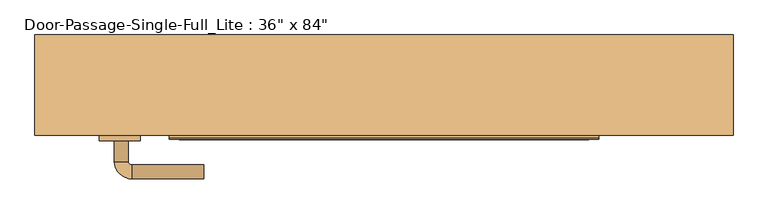
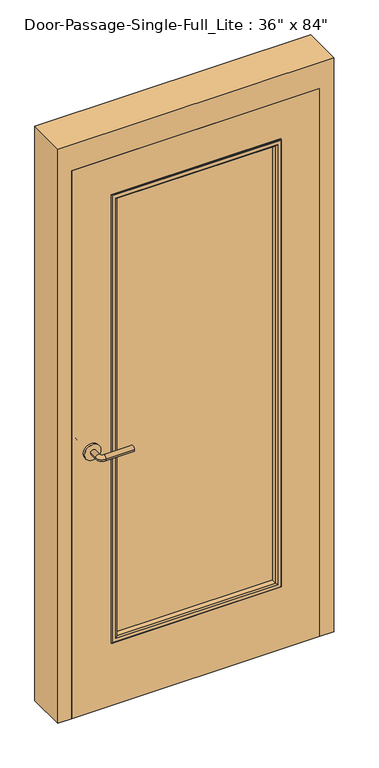
"""IFC4 building model written with IfcOpenShell, lengths in millimetres: door geometry."""

import ifcopenshell
import ifcopenshell.guid

model = None  # the IFC model being written
_history = None  # IfcOwnerHistory: only IFC2X3 demands one
_inside = {}  # id of a spatial element -> (the spatial element, [elements in it])
_under = {}  # id of a project, library or spatial element -> (it, [spatial elements below it])
_declared = {}  # id of a project -> (the project, [libraries it declares])
_typed = {}  # id of a type object -> (the type object, [elements of that type])
_made_of = {}  # id of a material, layer set ... -> (it, [elements and type objects made of it])


def new_model(schema):
    """Start an empty IFC model of exactly this schema.

    Asked for "IFC4X3", IfcOpenShell would pick the latest addendum, in which some entities
    have other attributes; the version numbers below select the first issue.
    IFC2X3 requires an IfcOwnerHistory on every rooted entity: one is made here for all.
    """
    global model, _history
    if schema == "IFC4X3":
        model = ifcopenshell.file(schema_version=(4, 3, 0, 0))
    else:
        model = ifcopenshell.file(schema=schema)
    _inside.clear()
    _under.clear()
    _declared.clear()
    _typed.clear()
    _made_of.clear()
    _history = None
    if model.schema == "IFC2X3":
        org = make("IfcOrganization", Name="unknown")
        user = make(
            "IfcPersonAndOrganization",
            ThePerson=make("IfcPerson", FamilyName="unknown"),
            TheOrganization=org,
        )
        app = make(
            "IfcApplication",
            ApplicationDeveloper=org,
            Version="unknown",
            ApplicationFullName="unknown",
            ApplicationIdentifier="unknown",
        )
        _history = make(
            "IfcOwnerHistory",
            OwningUser=user,
            OwningApplication=app,
            ChangeAction="ADDED",
            CreationDate=0,
        )
    return model


def make(cls, **values):
    """One entity of the class cls with the attributes given. An attribute that is None is left unset."""
    return model.create_entity(
        cls, **{name: value for name, value in values.items() if value is not None}
    )


def rooted(cls, **values):
    """An entity with a GlobalId (a new one), such as an element, a storey or a relation."""
    return make(cls, GlobalId=ifcopenshell.guid.new(), OwnerHistory=_history, **values)


def si_unit(unit_type, name, prefix=None):
    """IfcSIUnit, for example si_unit("LENGTHUNIT", "METRE", prefix="MILLI")."""
    return make("IfcSIUnit", UnitType=unit_type, Prefix=prefix, Name=name)


def assignment(units):
    """IfcUnitAssignment: the units of a project."""
    return None if units is None else make("IfcUnitAssignment", Units=units)


def point(xyz):
    """IfcCartesianPoint."""
    return None if xyz is None else make("IfcCartesianPoint", Coordinates=xyz)


def direction(xyz):
    """IfcDirection."""
    return None if xyz is None else make("IfcDirection", DirectionRatios=xyz)


def frame(location, z_axis=None, x_axis=None):
    """IfcAxis2Placement3D, a coordinate frame: its origin and axes. An axis left out is left unset."""
    return make(
        "IfcAxis2Placement3D",
        Location=point(location),
        Axis=direction(z_axis),
        RefDirection=direction(x_axis),
    )


def frame_2d(location, x_axis=None):
    """IfcAxis2Placement2D, a coordinate frame in the plane: its origin and x axis."""
    return make(
        "IfcAxis2Placement2D", Location=point(location), RefDirection=direction(x_axis)
    )


def origin():
    """The frame at (0, 0, 0) with its axes left unset."""
    return frame((0.0, 0.0, 0.0))


def place(relative_to, where):
    """IfcLocalPlacement: puts the frame where relative to a parent placement (None: the world)."""
    return make(
        "IfcLocalPlacement", PlacementRelTo=relative_to, RelativePlacement=where
    )


def context(
    kind, dimensions, precision=None, world=None, true_north=None, identifier=None
):
    """IfcGeometricRepresentationContext, for example the 3D "Model" context."""
    return make(
        "IfcGeometricRepresentationContext",
        ContextIdentifier=identifier,
        ContextType=kind,
        CoordinateSpaceDimension=dimensions,
        Precision=precision,
        WorldCoordinateSystem=world,
        TrueNorth=true_north,
    )


def project(units=None, contexts=None):
    """IfcProject with its units and contexts."""
    return rooted(
        "IfcProject",
        Name="project",
        RepresentationContexts=contexts,
        UnitsInContext=assignment(units),
    )


def spatial(cls, under=None, at=None, **own):
    """A site, building, storey or space (cls), placed at a placement, below another one or the project."""
    s = rooted(cls, ObjectPlacement=at, **own)
    if under is not None:
        _under.setdefault(under.id(), (under, []))[1].append(s)
    return s


def polyline(points):
    """IfcPolyline through the points."""
    return make("IfcPolyline", Points=[point(p) for p in points])


def circle_curve(where, radius):
    """IfcCircle in the frame where."""
    return make("IfcCircle", Position=where, Radius=radius)


def ellipse_curve(where, semi_axis1, semi_axis2):
    """IfcEllipse in the frame where."""
    return make(
        "IfcEllipse", Position=where, SemiAxis1=semi_axis1, SemiAxis2=semi_axis2
    )


def trimmed(basis, trim1, trim2, sense, master):
    """IfcTrimmedCurve: the piece of a basis curve between two trims."""
    return make(
        "IfcTrimmedCurve",
        BasisCurve=basis,
        Trim1=trim1,
        Trim2=trim2,
        SenseAgreement=sense,
        MasterRepresentation=master,
    )


def segment(curve, same_sense, transition):
    """IfcCompositeCurveSegment."""
    return make(
        "IfcCompositeCurveSegment",
        Transition=transition,
        SameSense=same_sense,
        ParentCurve=curve,
    )


def composite_curve(segments, self_intersect=None):
    """IfcCompositeCurve: segments joined end to end."""
    return make("IfcCompositeCurve", Segments=segments, SelfIntersect=self_intersect)


def outline(outer, holes=None, kind="AREA"):
    """IfcArbitraryClosedProfileDef: a profile drawn as a closed curve; with holes, ...WithVoids."""
    if holes is None:
        return make("IfcArbitraryClosedProfileDef", ProfileType=kind, OuterCurve=outer)
    return make(
        "IfcArbitraryProfileDefWithVoids",
        ProfileType=kind,
        OuterCurve=outer,
        InnerCurves=holes,
    )


def extrude(swept, where, along, depth):
    """IfcExtrudedAreaSolid: the profile swept, set in the frame where, extruded along a direction by depth."""
    return make(
        "IfcExtrudedAreaSolid",
        SweptArea=swept,
        Position=where,
        ExtrudedDirection=direction(along),
        Depth=depth,
    )


def faces_of(points, faces, orient=None, outer=None):
    """IfcFace entities. A face is a list of loops; a loop is a list of indices into points, from 0.

    orient and outer hold one flag for each loop. By default every Orientation is true, the
    first loop of a face is its IfcFaceOuterBound and the others are IfcFaceBound.
    """
    made = []
    for i, loops in enumerate(faces):
        bounds = []
        for j, loop in enumerate(loops):
            is_outer = j == 0 if outer is None else outer[i][j]
            bounds.append(
                make(
                    "IfcFaceOuterBound" if is_outer else "IfcFaceBound",
                    Bound=make("IfcPolyLoop", Polygon=[points[k] for k in loop]),
                    Orientation=True if orient is None else orient[i][j],
                )
            )
        made.append(make("IfcFace", Bounds=bounds))
    return made


def faceted_brep(points, faces, orient=None, outer=None, voids=None):
    """IfcFacetedBrep: a solid bounded by flat faces; with voids (closed shells), ...WithVoids."""
    shared = [point(p) for p in points]
    hull = make("IfcClosedShell", CfsFaces=faces_of(shared, faces, orient, outer))
    if voids is None:
        return make("IfcFacetedBrep", Outer=hull)
    return make(
        "IfcFacetedBrepWithVoids",
        Outer=hull,
        Voids=[
            make(cls, CfsFaces=faces_of(shared, fs, o, b)) for cls, fs, o, b in voids
        ],
    )


def shape(context_of_items, identifier, shape_type, items):
    """IfcShapeRepresentation: the items that make up one representation, for example the "Body"."""
    return make(
        "IfcShapeRepresentation",
        ContextOfItems=context_of_items,
        RepresentationIdentifier=identifier,
        RepresentationType=shape_type,
        Items=items,
    )


def source(mapping_origin, context_of_items, identifier, shape_type, items):
    """IfcRepresentationMap: a shape defined once, which mapped items show again and again."""
    return make(
        "IfcRepresentationMap",
        MappingOrigin=mapping_origin,
        MappedRepresentation=shape(context_of_items, identifier, shape_type, items),
    )


def transform(
    local_origin,
    x_axis=None,
    y_axis=None,
    z_axis=None,
    scale=None,
    scale2=None,
    scale3=None,
    uniform=True,
):
    """IfcCartesianTransformationOperator3D, or its non-uniform kind. x_axis, y_axis, z_axis: its Axis1, 2, 3."""
    if uniform:
        return make(
            "IfcCartesianTransformationOperator3D",
            Axis1=direction(x_axis),
            Axis2=direction(y_axis),
            LocalOrigin=point(local_origin),
            Scale=scale,
            Axis3=direction(z_axis),
        )
    return make(
        "IfcCartesianTransformationOperator3DnonUniform",
        Axis1=direction(x_axis),
        Axis2=direction(y_axis),
        LocalOrigin=point(local_origin),
        Scale=scale,
        Axis3=direction(z_axis),
        Scale2=scale2,
        Scale3=scale3,
    )


def mapped(mapping_source, mapping_target):
    """IfcMappedItem: shows the shape of a source again, moved by a transform."""
    return make(
        "IfcMappedItem", MappingSource=mapping_source, MappingTarget=mapping_target
    )


def made_of(thing, what):
    """Note that an element or type object is made of a material, layer set ...; save() writes the relation."""
    if what is not None:
        _made_of.setdefault(what.id(), (what, []))[1].append(thing)
    return thing


def element(
    cls,
    number,
    at=None,
    inside=None,
    cuts=None,
    type_object=None,
    material=None,
    context=None,
    identifier="Body",
    shape_type=None,
    held_by="IfcProductDefinitionShape",
    body=None,
    shapes=None,
    **own,
):
    """One element of the class cls, such as IfcWall. Its Tag is "e" and its number.

    at: its placement. inside: the storey or other place that contains it. cuts: it is an
    opening in that element (IfcRelVoidsElement). A single representation is given by context,
    identifier, shape_type and body (its items); several are given by shapes. held_by: the class
    of the entity that holds the representations. save() writes the other relations.
    """
    e = rooted(cls, Tag="e%d" % number, ObjectPlacement=at, **own)
    if body is not None:
        shapes = [shape(context, identifier, shape_type, body)]
    if shapes is not None:
        e.Representation = make(held_by, Representations=shapes)
    if inside is not None:
        _inside.setdefault(inside.id(), (inside, []))[1].append(e)
    if cuts is not None:
        rooted(
            "IfcRelVoidsElement", RelatingBuildingElement=cuts, RelatedOpeningElement=e
        )
    if type_object is not None:
        _typed.setdefault(type_object.id(), (type_object, []))[1].append(e)
    return made_of(e, material)


def aggregate(whole, parts):
    """IfcRelAggregates: a whole, such as a stair, and the parts it consists of."""
    return rooted("IfcRelAggregates", RelatingObject=whole, RelatedObjects=parts)


def save(model, path):
    """Write the relations noted so far, then the file.

    IfcRelAggregates (storeys below a building ...), IfcRelContainedInSpatialStructure (elements
    in a storey), IfcRelDefinesByType, IfcRelAssociatesMaterial and IfcRelDeclares: one each for
    every whole, place, type object, material and project.
    """
    for whole, parts in _under.values():
        aggregate(whole, parts)
    for where, things in _inside.values():
        rooted(
            "IfcRelContainedInSpatialStructure",
            RelatedElements=things,
            RelatingStructure=where,
        )
    for kind, things in _typed.values():
        rooted("IfcRelDefinesByType", RelatedObjects=things, RelatingType=kind)
    for what, things in _made_of.values():
        rooted("IfcRelAssociatesMaterial", RelatedObjects=things, RelatingMaterial=what)
    for by, libraries in _declared.values():
        rooted("IfcRelDeclares", RelatingContext=by, RelatedDefinitions=libraries)
    model.write(path)


def plane_surface(at):
    """IfcPlane: the flat surface through the origin of the frame at, square to its z axis."""
    return make("IfcPlane", Position=at)


def cylinder_surface(at, radius):
    """IfcCylindricalSurface: all points at the distance radius from the z axis of the frame at."""
    return make("IfcCylindricalSurface", Position=at, Radius=radius)


def revolved_surface(curve, axis_point, axis_direction):
    """IfcSurfaceOfRevolution: the curve turned about the line through axis_point along axis_direction."""
    return make(
        "IfcSurfaceOfRevolution",
        SweptCurve=make("IfcArbitraryOpenProfileDef", ProfileType="CURVE", Curve=curve),
        AxisPosition=make("IfcAxis1Placement", Location=point(axis_point), Axis=direction(axis_direction)),
    )


def advanced_brep(points, edges, surfaces, faces):
    """IfcAdvancedBrep: a solid bounded by faces that lie on surfaces and meet in shared edges.

    An edge is (start, end): straight between two places in points (the first is 0);
    or (start, end, curve); or (start, end, curve, False) where it runs against its curve.
    A face is (place in surfaces, loops), or (place, loops, False) where it looks against
    its surface's normal. A loop lists edges by number (the first is 1), with a minus sign
    where the edge is run from its end to its start. The first loop is the outer one.
    """
    corners = [point(p) for p in points]
    vertices = [make("IfcVertexPoint", VertexGeometry=c) for c in corners]
    made = []
    for start, end, *more in edges:
        made.append(
            make(
                "IfcEdgeCurve",
                EdgeStart=vertices[start],
                EdgeEnd=vertices[end],
                EdgeGeometry=more[0] if more else make("IfcPolyline", Points=[corners[start], corners[end]]),
                SameSense=more[1] if len(more) > 1 else True,
            )
        )
    hull = []
    for where, loops, *sense in faces:
        bounds = []
        for j, loop in enumerate(loops):
            ring = [make("IfcOrientedEdge", EdgeElement=made[abs(k) - 1], Orientation=k > 0) for k in loop]
            bounds.append(
                make(
                    "IfcFaceOuterBound" if j == 0 else "IfcFaceBound",
                    Bound=make("IfcEdgeLoop", EdgeList=ring),
                    Orientation=True,
                )
            )
        hull.append(make("IfcAdvancedFace", Bounds=bounds, FaceSurface=surfaces[where], SameSense=sense[0] if sense else True))
    return make("IfcAdvancedBrep", Outer=make("IfcClosedShell", CfsFaces=hull))


def door_5fc50167(model_context):
    return source(origin(), model_context, "Body", "SolidModel", [
        advanced_brep(
        [(-392.190625, 9.5875, 1016.0), (-372.190625, 9.5875, 1016.0), (-392.190625, 39.5875, 1016.0), (-372.190625, 39.5875, 1016.0), (-367.190625, 44.5875, 1016.0), (-367.190625, 64.5875, 1016.0), (-262.190625, 64.5875, 1016.0), (-262.190625, 44.5875, 1016.0)],
        [
            (0, 1, circle_curve(frame((-382.190625, 9.5875, 1016.0), z_axis=(0.0, -1.0, 0.0), x_axis=(1.0, 0.0, 0.0)), 10.0)),
            (1, 0, circle_curve(frame((-382.190625, 9.5875, 1016.0), z_axis=(0.0, -1.0, 0.0), x_axis=(1.0, 0.0, 0.0)), 10.0)),
            (0, 2),
            (2, 3, circle_curve(frame((-382.190625, 39.5875, 1016.0), z_axis=(0.0, -1.0, 0.0), x_axis=(1.0, 0.0, 0.0)), 10.0)),
            (3, 1),
            (3, 2, circle_curve(frame((-382.190625, 39.5875, 1016.0), z_axis=(0.0, -1.0, 0.0), x_axis=(1.0, 0.0, 0.0)), 10.0)),
            (4, 3, circle_curve(frame((-367.190625, 39.5875, 1016.0), z_axis=(0.0, 0.0, 1.0), x_axis=(-1.0, 0.0, 0.0)), 5.0)),
            (2, 5, circle_curve(frame((-367.190625, 39.5875, 1016.0), z_axis=(0.0, 0.0, -1.0), x_axis=(-1.0, 0.0, 0.0)), 25.0)),
            (5, 4, circle_curve(frame((-367.190625, 54.5875, 1016.0), z_axis=(-1.0, 0.0, 0.0), x_axis=(0.0, -1.0, 0.0)), 10.0)),
            (4, 5, circle_curve(frame((-367.190625, 54.5875, 1016.0), z_axis=(-1.0, 0.0, 0.0), x_axis=(0.0, -1.0, 0.0)), 10.0)),
            (6, 7, circle_curve(frame((-262.190625, 54.5875, 1016.0), z_axis=(1.0, 0.0, 0.0), x_axis=(0.0, -1.0, 0.0)), 10.0)),
            (7, 6, circle_curve(frame((-262.190625, 54.5875, 1016.0), z_axis=(1.0, 0.0, 0.0), x_axis=(0.0, -1.0, 0.0)), 10.0)),
            (5, 6),
            (7, 4),
        ],
        [
            plane_surface(frame((-382.190625, 9.5875, 1016.0), z_axis=(0.0, -1.0, 0.0), x_axis=(0.0, 0.0, 1.0))),
            cylinder_surface(frame((-382.190625, 9.5875, 1016.0), z_axis=(0.0, -1.0, 0.0), x_axis=(1.0, 0.0, 0.0)), 10.0),
            revolved_surface(trimmed(ellipse_curve(frame((-382.190625, 39.5875, 1016.0), z_axis=(0.0, -1.0, 0.0), x_axis=(1.0, 0.0, 0.0)), 10.0, 10.0), [point((-392.190625, 39.5875, 1016.0))], [point((-372.190625, 39.5875, 1016.0))], True, "CARTESIAN"), (-367.190625, 39.5875, 1016.0), (0.0, 0.0, -1.0)),
            revolved_surface(trimmed(ellipse_curve(frame((-382.190625, 39.5875, 1016.0), z_axis=(0.0, -1.0, 0.0), x_axis=(1.0, 0.0, 0.0)), 10.0, 10.0), [point((-372.190625, 39.5875, 1016.0))], [point((-392.190625, 39.5875, 1016.0))], True, "CARTESIAN"), (-367.190625, 39.5875, 1016.0), (0.0, 0.0, -1.0)),
            plane_surface(frame((-262.190625, 54.5875, 1016.0), z_axis=(1.0, 0.0, 0.0), x_axis=(0.0, 0.0, 1.0))),
            cylinder_surface(frame((-367.190625, 54.5875, 1016.0), z_axis=(-1.0, 0.0, 0.0), x_axis=(0.0, -1.0, 0.0)), 10.0),
        ],
        [
            (0, [[1, 2]]),
            (1, [[-1, 3, 4, 5]]),
            (1, [[-2, -5, 6, -3]]),
            (2, [[7, -4, 8, 9]]),
            (3, [[-8, -6, -7, 10]]),
            (4, [[11, 12]]),
            (5, [[-9, 13, -12, 14]]),
            (5, [[-10, -14, -11, -13]]),
        ],
    ),
        extrude(outline(composite_curve([segment(trimmed(circle_curve(frame_2d((1016.0, -384.690625)), 30.0), [point((1016.0, -414.690625))], [point((1016.0, -354.690625))], False, "CARTESIAN"), True, "CONTINUOUS"), segment(trimmed(circle_curve(frame_2d((1016.0, -384.690625)), 30.0), [point((1016.0, -354.690625))], [point((1016.0, -414.690625))], False, "CARTESIAN"), True, "CONTINUOUS")], self_intersect=False)), frame((0.0, 1.5875, 0.0), z_axis=(0.0, 1.0, 0.0), x_axis=(0.0, 0.0, 1.0)), (0.0, 0.0, 1.0), 8.0),
        advanced_brep(
        [(-392.190625, -50.8625, 1016.0), (-372.190625, -50.8625, 1016.0), (-372.190625, -80.8625, 1016.0), (-392.190625, -80.8625, 1016.0), (-367.190625, -85.8625, 1016.0), (-367.190625, -105.8625, 1016.0), (-262.190625, -105.8625, 1016.0), (-262.190625, -85.8625, 1016.0)],
        [
            (0, 1, circle_curve(frame((-382.190625, -50.8625, 1016.0), z_axis=(0.0, 1.0, 0.0), x_axis=(1.0, 0.0, 0.0)), 10.0)),
            (1, 0, circle_curve(frame((-382.190625, -50.8625, 1016.0), z_axis=(0.0, 1.0, 0.0), x_axis=(1.0, 0.0, 0.0)), 10.0)),
            (1, 2),
            (2, 3, circle_curve(frame((-382.190625, -80.8625, 1016.0), z_axis=(0.0, 1.0, 0.0), x_axis=(1.0, 0.0, 0.0)), 10.0)),
            (3, 0),
            (3, 2, circle_curve(frame((-382.190625, -80.8625, 1016.0), z_axis=(0.0, 1.0, 0.0), x_axis=(1.0, 0.0, 0.0)), 10.0)),
            (4, 5, circle_curve(frame((-367.190625, -95.8625, 1016.0), z_axis=(-1.0, 0.0, 0.0), x_axis=(0.0, 1.0, 0.0)), 10.0)),
            (5, 3, circle_curve(frame((-367.190625, -80.8625, 1016.0), z_axis=(0.0, 0.0, -1.0), x_axis=(-1.0, 0.0, 0.0)), 25.0)),
            (2, 4, circle_curve(frame((-367.190625, -80.8625, 1016.0), z_axis=(0.0, 0.0, 1.0), x_axis=(-1.0, 0.0, 0.0)), 5.0)),
            (5, 4, circle_curve(frame((-367.190625, -95.8625, 1016.0), z_axis=(-1.0, 0.0, 0.0), x_axis=(0.0, 1.0, 0.0)), 10.0)),
            (6, 7, circle_curve(frame((-262.190625, -95.8625, 1016.0), z_axis=(1.0, 0.0, 0.0), x_axis=(0.0, 1.0, 0.0)), 10.0)),
            (7, 6, circle_curve(frame((-262.190625, -95.8625, 1016.0), z_axis=(1.0, 0.0, 0.0), x_axis=(0.0, 1.0, 0.0)), 10.0)),
            (4, 7),
            (6, 5),
        ],
        [
            plane_surface(frame((-382.190625, -50.8625, 1016.0), z_axis=(0.0, 1.0, 0.0), x_axis=(0.0, 0.0, 1.0))),
            cylinder_surface(frame((-382.190625, -50.8625, 1016.0), z_axis=(0.0, 1.0, 0.0), x_axis=(1.0, 0.0, 0.0)), 10.0),
            revolved_surface(trimmed(ellipse_curve(frame((-382.190625, -80.8625, 1016.0), z_axis=(0.0, -1.0, 0.0), x_axis=(1.0, 0.0, 0.0)), 10.0, 10.0), [point((-392.190625, -80.8625, 1016.0))], [point((-372.190625, -80.8625, 1016.0))], True, "CARTESIAN"), (-367.190625, -80.8625, 1016.0), (0.0, 0.0, -1.0)),
            revolved_surface(trimmed(ellipse_curve(frame((-382.190625, -80.8625, 1016.0), z_axis=(0.0, -1.0, 0.0), x_axis=(1.0, 0.0, 0.0)), 10.0, 10.0), [point((-372.190625, -80.8625, 1016.0))], [point((-392.190625, -80.8625, 1016.0))], True, "CARTESIAN"), (-367.190625, -80.8625, 1016.0), (0.0, 0.0, -1.0)),
            plane_surface(frame((-262.190625, -95.8625, 1016.0), z_axis=(1.0, 0.0, 0.0), x_axis=(0.0, 0.0, 1.0))),
            cylinder_surface(frame((-367.190625, -95.8625, 1016.0), z_axis=(-1.0, 0.0, 0.0), x_axis=(0.0, 1.0, 0.0)), 10.0),
        ],
        [
            (0, [[1, 2]]),
            (1, [[3, 4, 5, -2]]),
            (1, [[-5, 6, -3, -1]]),
            (2, [[7, 8, -4, 9]]),
            (3, [[10, -9, -6, -8]]),
            (4, [[11, 12]]),
            (5, [[13, -11, 14, -7]]),
            (5, [[-14, -12, -13, -10]]),
        ],
    ),
        extrude(outline(composite_curve([segment(trimmed(circle_curve(frame_2d((1016.0, -384.690625)), 30.0), [point((1016.0, -414.690625))], [point((1016.0, -354.690625))], False, "CARTESIAN"), True, "CONTINUOUS"), segment(trimmed(circle_curve(frame_2d((1016.0, -384.690625)), 30.0), [point((1016.0, -354.690625))], [point((1016.0, -414.690625))], False, "CARTESIAN"), True, "CONTINUOUS")], self_intersect=False)), frame((0.0, -50.8625, 0.0), z_axis=(0.0, 1.0, 0.0), x_axis=(0.0, 0.0, 1.0)), (0.0, 0.0, 1.0), 8.0),
        extrude(outline(polyline([(304.8, -17.4625), (304.8, -23.8125), (-304.8, -23.8125), (-304.8, -17.4625), (304.8, -17.4625)])), frame((0.0, 0.0, 254.0), z_axis=(0.0, 0.0, 1.0), x_axis=(1.0, 0.0, 0.0)), (0.0, 0.0, 1.0), 1727.2),
        faceted_brep([(457.2, 6.35, 0.0), (441.325, 6.35, 0.0), (441.325, 53.975, 0.0), (457.2, 53.975, 0.0), (457.2, 103.1875, 0.0), (508.0, 103.1875, 0.0), (508.0, -42.8625, 0.0), (457.2, -42.8625, 0.0), (457.2, -42.8625, 2133.6), (457.2, 6.35, 2133.6), (508.0, -42.8625, 2235.2), (-508.0, -42.8625, 2235.2), (-508.0, -42.8625, 0.0), (-457.2, -42.8625, 0.0), (-457.2, -42.8625, 2133.6), (508.0, 103.1875, 2235.2), (457.2, 103.1875, 2133.6), (-457.2, 103.1875, 2133.6), (-457.2, 103.1875, 0.0), (-508.0, 103.1875, 0.0), (-508.0, 103.1875, 2235.2), (457.2, 53.975, 2133.6), (441.325, 53.975, 2117.725), (-441.325, 53.975, 2117.725), (-441.325, 53.975, 0.0), (-457.2, 53.975, 0.0), (-457.2, 53.975, 2133.6), (441.325, 6.35, 2117.725), (-457.2, 6.35, 2133.6), (-457.2, 6.35, 0.0), (-441.325, 6.35, 0.0), (-441.325, 6.35, 2117.725)], [[[0, 1, 2, 3, 4, 5, 6, 7]], [[7, 8, 9, 0]], [[6, 10, 11, 12, 13, 14, 8, 7]], [[5, 15, 10, 6]], [[4, 16, 17, 18, 19, 20, 15, 5]], [[3, 21, 16, 4]], [[2, 22, 23, 24, 25, 26, 21, 3]], [[1, 27, 22, 2]], [[0, 9, 28, 29, 30, 31, 27, 1]], [[8, 14, 28, 9]], [[16, 21, 26, 17]], [[22, 27, 31, 23]], [[12, 19, 18, 25, 24, 30, 29, 13]], [[13, 29, 28, 14]], [[11, 20, 19, 12]], [[17, 26, 25, 18]], [[23, 31, 30, 24]], [[15, 20, 11, 10]]]),
        extrude(outline(polyline([(2133.6, -457.2), (0.0, -457.2), (0.0, 457.2), (2133.6, 457.2), (2133.6, -457.2)]), holes=[polyline([(1981.2, -304.8), (1981.2, 304.8), (254.0, 304.8), (254.0, -304.8), (1981.2, -304.8)])]), frame((0.0, -42.8625, 0.0), z_axis=(0.0, 1.0, 0.0), x_axis=(0.0, 0.0, 1.0)), (0.0, 0.0, 1.0), 44.45),
        advanced_brep(
        [(-304.8, -23.8125, 1981.2), (-304.8, -23.8125, 254.0), (-304.8, -42.8625, 254.0), (-304.8, -42.8625, 1981.2), (-292.8, -43.8625, 1969.2), (-292.8, -43.8625, 266.0), (-292.8, -23.8125, 266.0), (-292.8, -23.8125, 1969.2), (-297.8, -48.8625, 1974.2), (-297.8, -48.8625, 261.0), (-312.8, -46.8625, 1989.2), (-312.8, -46.8625, 246.0), (-310.8, -48.8625, 248.0), (-310.8, -48.8625, 1987.2), (-312.8, -42.8625, 1989.2), (-312.8, -42.8625, 246.0), (304.8, -23.8125, 254.0), (304.8, -42.8625, 254.0), (292.8, -43.8625, 266.0), (292.8, -23.8125, 266.0), (297.8, -48.8625, 261.0), (312.8, -46.8625, 246.0), (310.8, -48.8625, 248.0), (312.8, -42.8625, 246.0), (304.8, -23.8125, 1981.2), (304.8, -42.8625, 1981.2), (292.8, -43.8625, 1969.2), (292.8, -23.8125, 1969.2), (297.8, -48.8625, 1974.2), (312.8, -46.8625, 1989.2), (310.8, -48.8625, 1987.2), (312.8, -42.8625, 1989.2)],
        [
            (0, 1),
            (1, 2),
            (2, 3),
            (3, 0),
            (4, 5),
            (5, 6),
            (6, 7),
            (7, 4),
            (8, 9),
            (9, 5, ellipse_curve(frame((-297.8, -43.8625, 261.0), z_axis=(-0.7071067811865475, 0.0, 0.7071067811865475), x_axis=(0.7071067811865474, 0.0, 0.7071067811865476)), 7.0710678, 5.0)),
            (4, 8, ellipse_curve(frame((-297.8, -43.8625, 1974.2), z_axis=(-0.7071067811865475, 0.0, -0.7071067811865475), x_axis=(-0.7071067811865474, 0.0, 0.7071067811865476)), 7.0710678, 5.0)),
            (10, 11),
            (11, 12, ellipse_curve(frame((-310.8, -46.8625, 248.0), z_axis=(-0.7071067811865475, 0.0, 0.7071067811865475), x_axis=(0.7071067811865474, 0.0, 0.7071067811865476)), 2.8284271, 2.0)),
            (12, 13),
            (13, 10, ellipse_curve(frame((-310.8, -46.8625, 1987.2), z_axis=(-0.7071067811865475, 0.0, -0.7071067811865475), x_axis=(-0.7071067811865474, 0.0, 0.7071067811865476)), 2.8284271, 2.0)),
            (14, 15),
            (15, 11),
            (10, 14),
            (1, 16),
            (16, 17),
            (17, 2),
            (5, 18),
            (18, 19),
            (19, 6),
            (9, 20),
            (20, 18, ellipse_curve(frame((297.8, -43.8625, 261.0), z_axis=(-0.7071067811865475, 0.0, -0.7071067811865475), x_axis=(-0.7071067811865476, 0.0, 0.7071067811865474)), 7.0710678, 5.0)),
            (11, 21),
            (21, 22, ellipse_curve(frame((310.8, -46.8625, 248.0), z_axis=(-0.7071067811865475, 0.0, -0.7071067811865475), x_axis=(-0.7071067811865476, 0.0, 0.7071067811865474)), 2.8284271, 2.0)),
            (22, 12),
            (15, 23),
            (23, 21),
            (16, 24),
            (24, 25),
            (25, 17),
            (18, 26),
            (26, 27),
            (27, 19),
            (20, 28),
            (28, 26, ellipse_curve(frame((297.8, -43.8625, 1974.2), z_axis=(0.7071067811865475, 0.0, -0.7071067811865475), x_axis=(-0.7071067811865474, 0.0, -0.7071067811865476)), 7.0710678, 5.0)),
            (21, 29),
            (29, 30, ellipse_curve(frame((310.8, -46.8625, 1987.2), z_axis=(0.7071067811865475, 0.0, -0.7071067811865475), x_axis=(-0.7071067811865474, 0.0, -0.7071067811865476)), 2.8284271, 2.0)),
            (30, 22),
            (23, 31),
            (31, 29),
            (14, 31),
            (25, 3),
            (24, 0),
            (27, 7),
            (26, 4),
            (28, 8),
            (30, 13),
            (29, 10),
        ],
        [
            plane_surface(frame((-304.8, -42.8625, 1981.2), z_axis=(-1.0, 0.0, 0.0), x_axis=(0.0, 0.0, -1.0))),
            plane_surface(frame((-292.8, -23.8125, 1969.2), z_axis=(1.0, 0.0, 0.0), x_axis=(0.0, 0.0, -1.0))),
            cylinder_surface(frame((-297.8, -43.8625, 1981.2), z_axis=(0.0, 0.0, 1.0), x_axis=(-1.0, 0.0, 0.0)), 5.0),
            cylinder_surface(frame((-310.8, -46.8625, 1981.2), z_axis=(0.0, 0.0, 1.0), x_axis=(-1.0, 0.0, 0.0)), 2.0),
            plane_surface(frame((-312.8, -46.8625, 1989.2), z_axis=(-1.0, 0.0, 0.0), x_axis=(0.0, 0.0, -1.0))),
            plane_surface(frame((-304.8, -42.8625, 254.0), z_axis=(0.0, 0.0, -1.0), x_axis=(1.0, 0.0, 0.0))),
            plane_surface(frame((-292.8, -23.8125, 266.0), z_axis=(0.0, 0.0, 1.0), x_axis=(1.0, 0.0, 0.0))),
            cylinder_surface(frame((-304.8, -43.8625, 261.0), z_axis=(-1.0, 0.0, 0.0), x_axis=(0.0, 0.0, -1.0)), 5.0),
            cylinder_surface(frame((-304.8, -46.8625, 248.0), z_axis=(-1.0, 0.0, 0.0), x_axis=(0.0, 0.0, -1.0)), 2.0),
            plane_surface(frame((-312.8, -46.8625, 246.0), z_axis=(0.0, 0.0, -1.0), x_axis=(1.0, 0.0, 0.0))),
            plane_surface(frame((304.8, -42.8625, 254.0), z_axis=(1.0, 0.0, 0.0), x_axis=(0.0, 0.0, 1.0))),
            plane_surface(frame((292.8, -23.8125, 266.0), z_axis=(-1.0, 0.0, 0.0), x_axis=(0.0, 0.0, 1.0))),
            cylinder_surface(frame((297.8, -43.8625, 254.0), z_axis=(0.0, 0.0, -1.0), x_axis=(1.0, 0.0, 0.0)), 5.0),
            cylinder_surface(frame((310.8, -46.8625, 254.0), z_axis=(0.0, 0.0, -1.0), x_axis=(1.0, 0.0, 0.0)), 2.0),
            plane_surface(frame((312.8, -46.8625, 246.0), z_axis=(1.0, 0.0, 0.0), x_axis=(0.0, 0.0, 1.0))),
            plane_surface(frame((312.8, -42.8625, 1989.2), z_axis=(0.0, 1.0, 0.0), x_axis=(-1.0, 0.0, 0.0))),
            plane_surface(frame((304.8, -42.8625, 1981.2), z_axis=(0.0, 0.0, 1.0), x_axis=(-1.0, 0.0, 0.0))),
            plane_surface(frame((304.8, -23.8125, 1981.2), z_axis=(0.0, 1.0, 0.0), x_axis=(-1.0, 0.0, 0.0))),
            plane_surface(frame((292.8, -23.8125, 1969.2), z_axis=(0.0, 0.0, -1.0), x_axis=(-1.0, 0.0, 0.0))),
            cylinder_surface(frame((304.8, -43.8625, 1974.2), z_axis=(1.0, 0.0, 0.0), x_axis=(0.0, 0.0, 1.0)), 5.0),
            plane_surface(frame((297.8, -48.8625, 1974.2), z_axis=(0.0, -1.0, 0.0), x_axis=(-1.0, 0.0, 0.0))),
            cylinder_surface(frame((304.8, -46.8625, 1987.2), z_axis=(1.0, 0.0, 0.0), x_axis=(0.0, 0.0, 1.0)), 2.0),
            plane_surface(frame((312.8, -46.8625, 1989.2), z_axis=(0.0, 0.0, 1.0), x_axis=(-1.0, 0.0, 0.0))),
        ],
        [
            (0, [[1, 2, 3, 4]]),
            (1, [[5, 6, 7, 8]]),
            (2, [[9, 10, -5, 11]]),
            (3, [[12, 13, 14, 15]]),
            (4, [[16, 17, -12, 18]]),
            (5, [[19, 20, 21, -2]]),
            (6, [[22, 23, 24, -6]]),
            (7, [[25, 26, -22, -10]]),
            (8, [[27, 28, 29, -13]]),
            (9, [[30, 31, -27, -17]]),
            (10, [[32, 33, 34, -20]]),
            (11, [[35, 36, 37, -23]]),
            (12, [[38, 39, -35, -26]]),
            (13, [[40, 41, 42, -28]]),
            (14, [[43, 44, -40, -31]]),
            (15, [[-16, 45, -43, -30], [-3, -21, -34, 46]]),
            (16, [[47, -4, -46, -33]]),
            (17, [[-1, -47, -32, -19], [-7, -24, -37, 48]]),
            (18, [[49, -8, -48, -36]]),
            (19, [[50, -11, -49, -39]]),
            (20, [[-14, -29, -42, 51], [-9, -50, -38, -25]]),
            (21, [[52, -15, -51, -41]]),
            (22, [[-45, -18, -52, -44]]),
        ],
    ),
        advanced_brep(
        [(-304.8, -17.4625, 254.0), (-304.8, -17.4625, 1981.2), (-304.8, 1.5875, 1981.2), (-304.8, 1.5875, 254.0), (-292.8, 2.5875, 266.0), (-292.8, 2.5875, 1969.2), (-292.8, -17.4625, 1969.2), (-292.8, -17.4625, 266.0), (-297.8, 7.5875, 261.0), (-297.8, 7.5875, 1974.2), (-312.8, 5.5875, 246.0), (-312.8, 5.5875, 1989.2), (-310.8, 7.5875, 1987.2), (-310.8, 7.5875, 248.0), (-312.8, 1.5875, 246.0), (-312.8, 1.5875, 1989.2), (304.8, -17.4625, 1981.2), (304.8, 1.5875, 1981.2), (292.8, 2.5875, 1969.2), (292.8, -17.4625, 1969.2), (297.8, 7.5875, 1974.2), (312.8, 5.5875, 1989.2), (310.8, 7.5875, 1987.2), (312.8, 1.5875, 1989.2), (304.8, -17.4625, 254.0), (304.8, 1.5875, 254.0), (292.8, 2.5875, 266.0), (292.8, -17.4625, 266.0), (297.8, 7.5875, 261.0), (312.8, 5.5875, 246.0), (310.8, 7.5875, 248.0), (312.8, 1.5875, 246.0)],
        [
            (0, 1),
            (1, 2),
            (2, 3),
            (3, 0),
            (4, 5),
            (5, 6),
            (6, 7),
            (7, 4),
            (8, 9),
            (9, 5, ellipse_curve(frame((-297.8, 2.5875, 1974.2), z_axis=(-0.7071067811865475, 0.0, -0.7071067811865475), x_axis=(0.7071067811865474, 0.0, -0.7071067811865476)), 7.0710678, 5.0)),
            (4, 8, ellipse_curve(frame((-297.8, 2.5875, 261.0), z_axis=(-0.7071067811865475, 0.0, 0.7071067811865475), x_axis=(-0.7071067811865474, 0.0, -0.7071067811865476)), 7.0710678, 5.0)),
            (10, 11),
            (11, 12, ellipse_curve(frame((-310.8, 5.5875, 1987.2), z_axis=(-0.7071067811865475, 0.0, -0.7071067811865475), x_axis=(0.7071067811865474, 0.0, -0.7071067811865476)), 2.8284271, 2.0)),
            (12, 13),
            (13, 10, ellipse_curve(frame((-310.8, 5.5875, 248.0), z_axis=(-0.7071067811865475, 0.0, 0.7071067811865475), x_axis=(-0.7071067811865474, 0.0, -0.7071067811865476)), 2.8284271, 2.0)),
            (14, 15),
            (15, 11),
            (10, 14),
            (1, 16),
            (16, 17),
            (17, 2),
            (5, 18),
            (18, 19),
            (19, 6),
            (9, 20),
            (20, 18, ellipse_curve(frame((297.8, 2.5875, 1974.2), z_axis=(-0.7071067811865475, 0.0, 0.7071067811865475), x_axis=(-0.7071067811865476, 0.0, -0.7071067811865474)), 7.0710678, 5.0)),
            (11, 21),
            (21, 22, ellipse_curve(frame((310.8, 5.5875, 1987.2), z_axis=(-0.7071067811865475, 0.0, 0.7071067811865475), x_axis=(-0.7071067811865476, 0.0, -0.7071067811865474)), 2.8284271, 2.0)),
            (22, 12),
            (15, 23),
            (23, 21),
            (16, 24),
            (24, 25),
            (25, 17),
            (18, 26),
            (26, 27),
            (27, 19),
            (20, 28),
            (28, 26, ellipse_curve(frame((297.8, 2.5875, 261.0), z_axis=(0.7071067811865475, 0.0, 0.7071067811865475), x_axis=(-0.7071067811865474, 0.0, 0.7071067811865476)), 7.0710678, 5.0)),
            (21, 29),
            (29, 30, ellipse_curve(frame((310.8, 5.5875, 248.0), z_axis=(0.7071067811865475, 0.0, 0.7071067811865475), x_axis=(-0.7071067811865474, 0.0, 0.7071067811865476)), 2.8284271, 2.0)),
            (30, 22),
            (23, 31),
            (31, 29),
            (14, 31),
            (25, 3),
            (24, 0),
            (27, 7),
            (26, 4),
            (28, 8),
            (30, 13),
            (29, 10),
        ],
        [
            plane_surface(frame((-304.8, 1.5875, 254.0), z_axis=(-1.0, 0.0, 0.0), x_axis=(0.0, 0.0, 1.0))),
            plane_surface(frame((-292.8, -17.4625, 266.0), z_axis=(1.0, 0.0, 0.0), x_axis=(0.0, 0.0, 1.0))),
            cylinder_surface(frame((-297.8, 2.5875, 254.0), z_axis=(0.0, 0.0, -1.0), x_axis=(-1.0, 0.0, 0.0)), 5.0),
            cylinder_surface(frame((-310.8, 5.5875, 254.0), z_axis=(0.0, 0.0, -1.0), x_axis=(-1.0, 0.0, 0.0)), 2.0),
            plane_surface(frame((-312.8, 5.5875, 246.0), z_axis=(-1.0, 0.0, 0.0), x_axis=(0.0, 0.0, 1.0))),
            plane_surface(frame((-304.8, 1.5875, 1981.2), z_axis=(0.0, 0.0, 1.0), x_axis=(1.0, 0.0, 0.0))),
            plane_surface(frame((-292.8, -17.4625, 1969.2), z_axis=(0.0, 0.0, -1.0), x_axis=(1.0, 0.0, 0.0))),
            cylinder_surface(frame((-304.8, 2.5875, 1974.2), z_axis=(-1.0, 0.0, 0.0), x_axis=(0.0, 0.0, 1.0)), 5.0),
            cylinder_surface(frame((-304.8, 5.5875, 1987.2), z_axis=(-1.0, 0.0, 0.0), x_axis=(0.0, 0.0, 1.0)), 2.0),
            plane_surface(frame((-312.8, 5.5875, 1989.2), z_axis=(0.0, 0.0, 1.0), x_axis=(1.0, 0.0, 0.0))),
            plane_surface(frame((304.8, 1.5875, 1981.2), z_axis=(1.0, 0.0, 0.0), x_axis=(0.0, 0.0, -1.0))),
            plane_surface(frame((292.8, -17.4625, 1969.2), z_axis=(-1.0, 0.0, 0.0), x_axis=(0.0, 0.0, -1.0))),
            cylinder_surface(frame((297.8, 2.5875, 1981.2), z_axis=(0.0, 0.0, 1.0), x_axis=(1.0, 0.0, 0.0)), 5.0),
            cylinder_surface(frame((310.8, 5.5875, 1981.2), z_axis=(0.0, 0.0, 1.0), x_axis=(1.0, 0.0, 0.0)), 2.0),
            plane_surface(frame((312.8, 5.5875, 1989.2), z_axis=(1.0, 0.0, 0.0), x_axis=(0.0, 0.0, -1.0))),
            plane_surface(frame((312.8, 1.5875, 246.0), z_axis=(0.0, -1.0, 0.0), x_axis=(-1.0, 0.0, 0.0))),
            plane_surface(frame((304.8, 1.5875, 254.0), z_axis=(0.0, 0.0, -1.0), x_axis=(-1.0, 0.0, 0.0))),
            plane_surface(frame((304.8, -17.4625, 254.0), z_axis=(0.0, -1.0, 0.0), x_axis=(-1.0, 0.0, 0.0))),
            plane_surface(frame((292.8, -17.4625, 266.0), z_axis=(0.0, 0.0, 1.0), x_axis=(-1.0, 0.0, 0.0))),
            cylinder_surface(frame((304.8, 2.5875, 261.0), z_axis=(1.0, 0.0, 0.0), x_axis=(0.0, 0.0, -1.0)), 5.0),
            plane_surface(frame((297.8, 7.5875, 261.0), z_axis=(0.0, 1.0, 0.0), x_axis=(-1.0, 0.0, 0.0))),
            cylinder_surface(frame((304.8, 5.5875, 248.0), z_axis=(1.0, 0.0, 0.0), x_axis=(0.0, 0.0, -1.0)), 2.0),
            plane_surface(frame((312.8, 5.5875, 246.0), z_axis=(0.0, 0.0, -1.0), x_axis=(-1.0, 0.0, 0.0))),
        ],
        [
            (0, [[1, 2, 3, 4]]),
            (1, [[5, 6, 7, 8]]),
            (2, [[9, 10, -5, 11]]),
            (3, [[12, 13, 14, 15]]),
            (4, [[16, 17, -12, 18]]),
            (5, [[19, 20, 21, -2]]),
            (6, [[22, 23, 24, -6]]),
            (7, [[25, 26, -22, -10]]),
            (8, [[27, 28, 29, -13]]),
            (9, [[30, 31, -27, -17]]),
            (10, [[32, 33, 34, -20]]),
            (11, [[35, 36, 37, -23]]),
            (12, [[38, 39, -35, -26]]),
            (13, [[40, 41, 42, -28]]),
            (14, [[43, 44, -40, -31]]),
            (15, [[-16, 45, -43, -30], [-3, -21, -34, 46]]),
            (16, [[47, -4, -46, -33]]),
            (17, [[-1, -47, -32, -19], [-7, -24, -37, 48]]),
            (18, [[49, -8, -48, -36]]),
            (19, [[50, -11, -49, -39]]),
            (20, [[-14, -29, -42, 51], [-9, -50, -38, -25]]),
            (21, [[52, -15, -51, -41]]),
            (22, [[-45, -18, -52, -44]]),
        ],
    ),
    ])


if __name__ == "__main__":
    model = new_model("IFC4")
    model_context = context("Model", 3, world=origin())
    ifc_project = project(units=[si_unit("LENGTHUNIT", "METRE", prefix="MILLI")], contexts=[model_context])
    site = spatial("IfcSite", under=ifc_project)
    building = spatial("IfcBuilding", under=site)
    placement = place(None, origin())
    door_shape = door_5fc50167(model_context)
    element("IfcDoor", 1, ObjectType="Door-Passage-Single-Full_Lite : 36\" x 84\"", at=placement, inside=building, context=model_context, shape_type="MappedRepresentation", body=[
        mapped(door_shape, transform((0.0, 0.0, 0.0), x_axis=(1.0, 0.0, 0.0), y_axis=(0.0, 1.0, 0.0), z_axis=(0.0, 0.0, 1.0))),
    ])
    save(model, "model.ifc")

# Revit data of these elements
# Type "Door-Passage-Single-Full_Lite : 36\" x 84\""
#   Type Mark = "52"
#   Assembly Code = "B2030100"
#   Analytic Construction = "Wooden"
#   Thickness = 0' - 1 3/4"
#   Thermal Resistance (R) = 2.5876 (h·ft²·°F)/BTU
#   Swing Angle [instance default] = 90.00°
#   Strike Height = 3' - 4"
#   Rough Width [instance default] = 3' - 4"
#   Rough Height [instance default] = 7' - 4"
#   MF Opening Height [instance default] = 0' - 4"
#   MF Opening Width [instance default] = 0' - 4"
#   Inset Calculate [instance default] = 0' - 4"
#   Masonry Inset [instance default] = 0' - 1"
#   Height = 7' - 0"
#   Width = 3' - 0"
#   Heat Transfer Coefficient (U) = 0.3865 BTU/(h·ft²·°F)
#   Masonry Frame Depth = 0' - 5 3/4"
#   Masonry Frame [instance default] = yes
#   Function = 1
#   Dry Wall Frame [instance default] = no
#   Panel Material = Wood - Birch
#   Glazing = Glass
#   Glass Stop Material = Metal - Paint Finish - Grey
#   Frame Material = Metal - Paint Finish - Grey
#   Door Handle Material = Aluminum
#   Visual Light Transmittance = 0
#   Solar Heat Gain Coefficient = 0
#   Wall Closure = (empty or 0)
# Element 1 (IfcDoor, "Door-Passage-Single-Full_Lite : 36\" x 84\"")
#   Materials on its faces: "Metal - Paint Finish - Grey", "Aluminum", "Wood - Birch", "Glass"
# Materials
#   "Wood - Birch": class "Wood", colour RGB 166 116 52, transparency 0, Cost = 0
#   "Glass": class "Glass", colour RGB 0 128 192, transparency 0.75, Description = "Soda Lime Glass", Cost = 0
#   "Metal - Paint Finish - Grey": class "Paint", colour RGB 104 104 104, transparency 0, Cost = 0
#   "Aluminum": class "Metal", colour RGB 247 247 247, transparency 0, Description = "Aluminum 6061", Cost = 0
